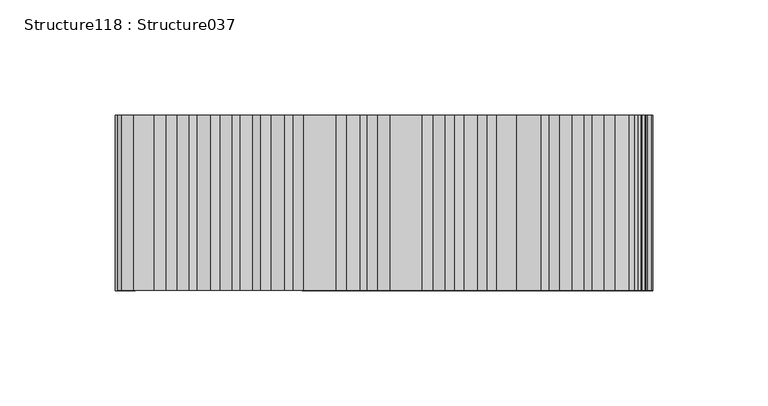
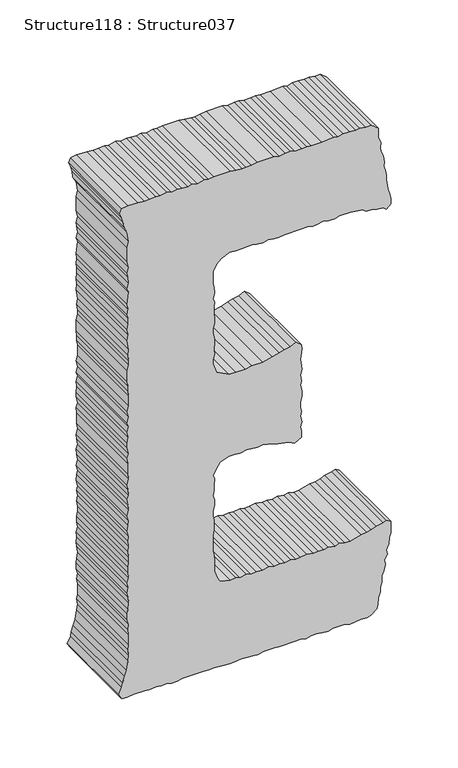
"""IFC4 building model written with IfcOpenShell, lengths in millimetres: proxy geometry, Structure118 : Structure037."""

from ifc_helpers import new_model, si_unit, frame, origin, place, context, project, spatial, polyline, outline, extrude, source, transform, mapped, element, save


def structure118_structure037_a706b3ca(model_context):
    return source(origin(), model_context, "Body", "SweptSolid", [
        extrude(outline(polyline([(3552.242032, -45108.9391366), (3556.3417965, -45103.663197), (3559.8671125, -45103.0887486), (3565.7094775, -45102.4966495), (3570.4109687, -45100.738003), (3574.5107332, -45100.738003), (3578.6104977, -45099.5714555), (3584.4689087, -45099.5714555), (3588.5702778, -45097.812809), (3593.8285667, -45096.6398431), (3598.5284533, -45097.22071), (3602.6298224, -45094.8779874), (3606.7295868, -45095.4716911), (3611.4134274, -45093.7034169), (3617.2718384, -45093.1193409), (3620.7971545, -45091.954398), (3625.472972, -45091.954398), (3631.3410106, -45091.954398), (3633.6821286, -45095.4716911), (3632.5155811, -45098.3968851), (3631.3410106, -45104.2536915), (3629.5984101, -45108.3550606), (3628.4158166, -45112.454825), (3627.8397636, -45117.1482932), (3625.472972, -45126.5159742), (3625.472972, -45131.2078378), (3626.6571701, -45135.9013059), (3625.472972, -45139.4169944), (3626.6571701, -45145.2673824), (3625.472972, -45149.3687515), (3626.0554434, -45154.0590104), (3625.472972, -45158.1603795), (3626.6571701, -45164.0187905), (3626.0554434, -45169.2947301), (3625.472972, -45173.3944946), (3626.6571701, -45177.5038867), (3625.472972, -45182.7621756), (3626.0554434, -45186.8715677), (3625.472972, -45191.5538037), (3626.6571701, -45196.2472718), (3625.472972, -45202.1056828), (3626.0554434, -45207.3816224), (3625.472972, -45212.0718813), (3626.6571701, -45215.590779), (3625.472972, -45221.441167), (3626.6571701, -45224.95846), (3626.0554434, -45229.640696), (3628.4158166, -45238.4355332), (3631.915459, -45240.7750466), (3638.9580681, -45243.1177691), (3648.9258713, -45243.1177691), (3654.1841602, -45243.7098682), (3657.7014533, -45244.2923396), (3671.7690209, -45244.2923396), (3677.0449604, -45243.7098682), (3685.8285655, -45243.7098682), (3689.3458585, -45244.2923396), (3694.029699, -45244.2923396), (3699.3136616, -45243.1177691), (3704.0135482, -45243.1177691), (3708.087639, -45244.2923396), (3712.2146818, -45243.7098682), (3716.8985223, -45243.7098682), (3722.7312597, -45243.1177691), (3726.2742264, -45244.2923396), (3733.8736333, -45240.1925751), (3736.2163558, -45238.4355332), (3739.1592005, -45230.8248941), (3739.1592005, -45225.5393269), (3738.5574738, -45221.441167), (3739.7416719, -45215.590779), (3739.1592005, -45212.0718813), (3738.5574738, -45206.2070519), (3739.1592005, -45202.1056828), (3737.400554, -45193.3204732), (3735.6146291, -45188.6302143), (3734.47536, -45182.7621756), (3733.2991849, -45178.6608065), (3730.9323932, -45174.5690651), (3734.47536, -45168.7010264), (3739.7416719, -45168.7010264), (3744.4158848, -45169.2947301), (3748.5429276, -45168.1201596), (3753.8012165, -45169.2947301), (3757.8753073, -45168.7010264), (3762.0023501, -45169.2947301), (3766.684586, -45169.2947301), (3771.3860772, -45168.1201596), (3776.6427615, -45168.1201596), (3781.9299333, -45169.2947301), (3785.4456218, -45168.7010264), (3791.3056374, -45169.2947301), (3795.960595, -45168.1201596), (3799.5051664, -45168.7010264), (3805.3459267, -45169.2947301), (3814.7296538, -45168.1201596), (3818.2309008, -45168.7010264), (3822.348316, -45173.3944946), (3820.015221, -45178.0863581), (3818.8310229, -45183.3542747), (3817.6741031, -45187.4556438), (3815.9154565, -45193.3204732), (3814.148787, -45201.5135838), (3814.148787, -45210.8973109), (3812.9726119, -45216.7476988), (3812.9726119, -45224.95846), (3813.5743386, -45230.8248941), (3818.8310229, -45241.3671456), (3827.6162325, -45244.2923396), (3831.1575946, -45244.2923396), (3835.8334121, -45243.1177691), (3840.5172527, -45243.7098682), (3845.8012153, -45243.1177691), (3849.8753061, -45243.1177691), (3855.1769193, -45244.2923396), (3859.2606378, -45244.2923396), (3863.9332461, -45243.1177691), (3868.0618934, -45243.1177691), (3873.3185778, -45243.7098682), (3878.5784713, -45243.7098682), (3883.2863809, -45243.1177691), (3886.2051565, -45244.2923396), (3891.5067697, -45243.1177691), (3896.763454, -45243.7098682), (3900.2887701, -45244.2923396), (3910.8310217, -45244.2923396), (3916.6653636, -45241.3671456), (3920.7908018, -45237.8514572), (3923.7079727, -45230.232795), (3923.1319197, -45224.95846), (3923.7079727, -45220.2649919), (3923.7079727, -45210.8973109), (3923.1319197, -45207.3816224), (3922.5494483, -45201.5135838), (3923.7079727, -45197.4122147), (3922.5494483, -45192.1459027), (3922.5494483, -45188.0461382), (3923.1319197, -45183.3542747), (3923.1319197, -45169.2947301), (3923.7079727, -45163.4347145), (3922.5494483, -45158.7524786), (3922.5494483, -45154.6527141), (3923.7079727, -45149.9592459), (3922.5494483, -45145.2673824), (3922.5494483, -45140.0010704), (3923.7079727, -45135.9013059), (3923.7079727, -45126.5159742), (3922.5494483, -45115.9721181), (3920.2067257, -45113.0485287), (3919.6066036, -45108.3550606), (3918.4480792, -45103.663197), (3917.8479571, -45098.3968851), (3915.5068392, -45095.4716911), (3919.6066036, -45091.954398), (3924.2888396, -45091.954398), (3928.4158823, -45092.538474), (3933.6741713, -45094.2971206), (3937.1930689, -45094.8779874), (3942.4770315, -45095.4716911), (3946.5511223, -45095.4716911), (3951.2606365, -45096.6398431), (3955.360401, -45097.812809), (3959.4617701, -45097.22071), (3965.3201811, -45098.3968851), (3969.994394, -45100.1555316), (3973.5197101, -45100.738003), (3977.6194746, -45100.1555316), (3983.4794902, -45102.4966495), (3988.1633307, -45102.4966495), (3991.6806238, -45102.4966495), (3996.390138, -45108.3550606), (3996.390138, -45113.0485287), (3996.9645864, -45118.3228637), (3996.390138, -45121.8401567), (3996.9645864, -45127.1064687), (3996.9645864, -45132.3840129), (3995.7803883, -45137.0758764), (3996.9645864, -45140.5835419), (3995.7803883, -45151.135421), (3995.7803883, -45159.9093984), (3996.390138, -45164.0187905), (3995.7803883, -45168.1201596), (3995.7803883, -45173.9881982), (3996.9645864, -45178.0863581), (3996.9645864, -45182.1861226), (3995.7803883, -45187.4556438), (3996.9645864, -45192.1459027), (3996.9645864, -45206.2070519), (3996.390138, -45211.4813869), (3995.7803883, -45216.1636228), (3995.7803883, -45219.100049), (3996.390138, -45224.95846), (3996.9645864, -45229.640696), (3996.9645864, -45243.7098682), (3996.390138, -45248.3921041), (3996.9645864, -45251.9093972), (3995.7803883, -45257.7597851), (3996.9645864, -45262.4532533), (3995.7803883, -45265.9689417), (3996.390138, -45271.2448813), (3996.390138, -45274.7605698), (3995.7803883, -45280.0300909), (3996.9645864, -45284.1282508), (3995.7803883, -45289.9962895), (3996.390138, -45293.5135825), (3995.7803883, -45298.7814991), (3995.7803883, -45303.463735), (3996.390138, -45308.7476976), (3996.390138, -45317.5329072), (3995.7803883, -45322.8088468), (3991.6806238, -45324.5658887), (3987.5792547, -45322.8088468), (3982.8793681, -45321.6342763), (3977.6194746, -45321.0405726), (3972.3627903, -45318.1153786), (3964.1343784, -45316.9488312), (3958.8776941, -45318.1153786), (3945.9766739, -45318.1153786), (3940.718385, -45316.9488312), (3935.4328178, -45318.1153786), (3931.9058971, -45317.5329072), (3926.0490907, -45316.9488312), (3921.3748778, -45318.1153786), (3917.8479571, -45316.9488312), (3907.3313793, -45318.1153786), (3902.6314927, -45317.5329072), (3897.9476522, -45318.1153786), (3894.4030808, -45317.5329072), (3889.7208449, -45317.5329072), (3884.4609514, -45318.1153786), (3879.7610648, -45317.5329072), (3874.5043805, -45318.1153786), (3866.3032469, -45316.9488312), (3861.0192843, -45317.5329072), (3855.7353217, -45316.9488312), (3852.2340747, -45316.9488312), (3846.9757858, -45318.1153786), (3836.9919366, -45318.1153786), (3832.8921721, -45317.5329072), (3828.2163546, -45317.5329072), (3824.1149855, -45316.9488312), (3814.7296538, -45316.9488312), (3810.0474179, -45318.1153786), (3804.7730829, -45316.9488312), (3799.5051664, -45318.1153786), (3795.960595, -45316.9488312), (3791.3056374, -45318.1153786), (3786.6298199, -45317.5329072), (3781.3282066, -45318.1153786), (3777.2444882, -45318.1153786), (3771.3860772, -45316.9488312), (3767.8607611, -45318.1153786), (3762.5848215, -45317.5329072), (3753.2171405, -45317.5329072), (3748.5429276, -45316.9488312), (3743.2332913, -45318.1153786), (3739.1592005, -45317.5329072), (3733.8736333, -45316.9488312), (3730.3563402, -45318.1153786), (3725.0996559, -45317.5329072), (3720.4158154, -45316.9488312), (3715.1302482, -45318.1153786), (3710.4560353, -45316.9488312), (3706.9130685, -45317.5329072), (3701.6547796, -45318.1153786), (3696.3884676, -45316.9488312), (3692.2710525, -45317.5329072), (3687.587212, -45316.9488312), (3682.8857208, -45317.5329072), (3677.6274319, -45316.9488312), (3672.9435914, -45316.9488312), (3668.8261762, -45317.5329072), (3663.5598643, -45317.5329072), (3658.8840468, -45316.9488312), (3654.7842823, -45318.1153786), (3650.1004418, -45317.5329072), (3645.4262289, -45318.1153786), (3641.2991861, -45317.5329072), (3636.0408972, -45316.9488312), (3630.7392839, -45317.5329072), (3626.6571701, -45318.1153786), (3621.3732075, -45318.1153786), (3616.69739, -45316.9488312), (3612.0135494, -45317.5329072), (3607.3393366, -45316.9488312), (3597.9540049, -45316.9488312), (3593.8285667, -45317.5329072), (3588.5702778, -45316.9488312), (3583.8864372, -45317.5329072), (3575.6853037, -45318.6978501), (3570.9854171, -45320.4661242), (3565.7094775, -45322.2151431), (3561.6257591, -45322.8088468), (3555.7416744, -45325.7324362), (3551.0658569, -45322.8088468), (3551.0658569, -45318.1153786), (3551.6675836, -45312.8490667), (3551.6675836, -45303.463735), (3551.0658569, -45299.3623659), (3551.6675836, -45293.5135825), (3551.0658569, -45288.821719), (3551.6675836, -45284.7203499), (3550.4833855, -45280.0300909), (3550.4833855, -45275.3446458), (3551.6675836, -45270.6608053), (3551.6675836, -45252.4934732), (3551.0658569, -45247.8112373), (3551.6675836, -45243.7098682), (3550.4833855, -45233.157989), (3550.4833855, -45229.0566199), (3551.0658569, -45223.782285), (3551.6675836, -45220.2649919), (3551.0658569, -45214.9986799), (3551.0658569, -45210.3052118), (3550.4833855, -45206.2070519), (3551.6675836, -45200.9391354), (3551.6675836, -45191.5538037), (3551.0658569, -45188.0461382), (3551.0658569, -45173.9881982), (3551.6675836, -45169.2947301), (3550.4833855, -45164.6028665), (3551.6675836, -45160.5031021), (3551.6675836, -45155.8176569), (3551.0658569, -45151.135421), (3550.4833855, -45145.2673824), (3551.6675836, -45141.7500893), (3551.6675836, -45131.2078378), (3550.4833855, -45127.1064687), (3551.6675836, -45117.7307646), (3551.0658569, -45112.454825), (3552.242032, -45108.9391366)])), frame((0.0, 247945.1599557, 0.0), z_axis=(0.0, 1.0, 0.0), x_axis=(0.0, 0.0, 1.0)), (0.0, 0.0, 1.0), 76.2),
    ])


if __name__ == "__main__":
    model = new_model("IFC4")
    model_context = context("Model", 3, world=origin())
    ifc_project = project(units=[si_unit("LENGTHUNIT", "METRE", prefix="MILLI")], contexts=[model_context])
    site = spatial("IfcSite", under=ifc_project)
    building = spatial("IfcBuilding", under=site)
    placement = place(None, origin())
    structure118_structure037_shape = structure118_structure037_a706b3ca(model_context)
    element("IfcBuildingElementProxy", 1, Name="Structure118 : Structure037", ObjectType="Structure118 : Structure037", at=placement, inside=building, context=model_context, shape_type="MappedRepresentation", body=[
        mapped(structure118_structure037_shape, transform((0.0, 0.0, 0.0), x_axis=(1.0, 0.0, 0.0), y_axis=(0.0, 1.0, 0.0), z_axis=(0.0, 0.0, 1.0))),
    ])
    save(model, "model.ifc")

# Revit data of these elements
# Type "Structure118 : Structure037"
#   NameOverride = "Structure037"
# Element 1 (IfcBuildingElementProxy, "Structure118 : Structure037")
#   Materials on its faces: "BRUSHED ALUM. LETTERING"
# Materials
#   "BRUSHED ALUM. LETTERING": class "Unassigned", colour RGB 169 181 186, transparency 0, Cost = 0
